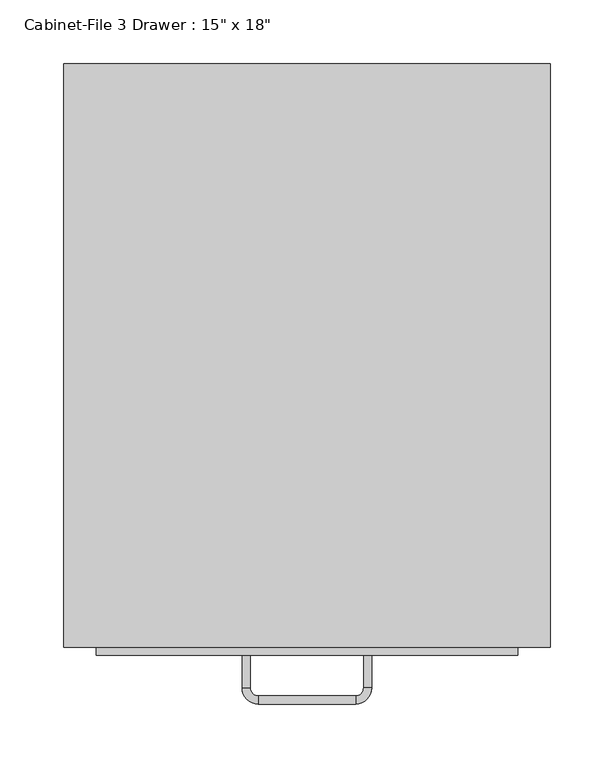
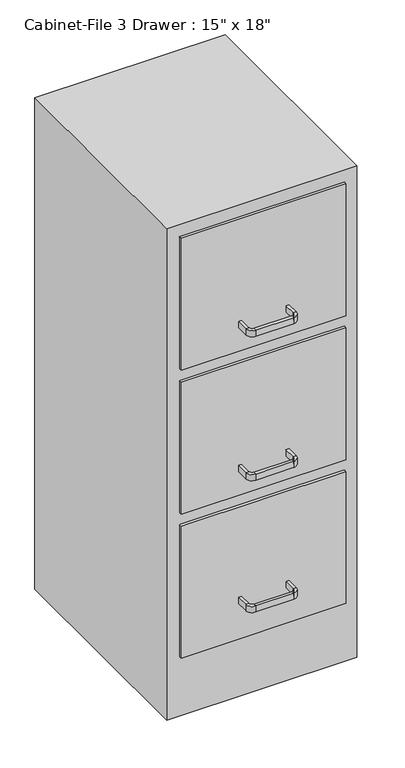
"""IFC4 building model written with IfcOpenShell, lengths in millimetres: furniture geometry."""

import ifcopenshell
import ifcopenshell.guid

model = None  # the IFC model being written
_history = None  # IfcOwnerHistory: only IFC2X3 demands one
_inside = {}  # id of a spatial element -> (the spatial element, [elements in it])
_under = {}  # id of a project, library or spatial element -> (it, [spatial elements below it])
_declared = {}  # id of a project -> (the project, [libraries it declares])
_typed = {}  # id of a type object -> (the type object, [elements of that type])
_made_of = {}  # id of a material, layer set ... -> (it, [elements and type objects made of it])


def new_model(schema):
    """Start an empty IFC model of exactly this schema.

    Asked for "IFC4X3", IfcOpenShell would pick the latest addendum, in which some entities
    have other attributes; the version numbers below select the first issue.
    IFC2X3 requires an IfcOwnerHistory on every rooted entity: one is made here for all.
    """
    global model, _history
    if schema == "IFC4X3":
        model = ifcopenshell.file(schema_version=(4, 3, 0, 0))
    else:
        model = ifcopenshell.file(schema=schema)
    _inside.clear()
    _under.clear()
    _declared.clear()
    _typed.clear()
    _made_of.clear()
    _history = None
    if model.schema == "IFC2X3":
        org = make("IfcOrganization", Name="unknown")
        user = make(
            "IfcPersonAndOrganization",
            ThePerson=make("IfcPerson", FamilyName="unknown"),
            TheOrganization=org,
        )
        app = make(
            "IfcApplication",
            ApplicationDeveloper=org,
            Version="unknown",
            ApplicationFullName="unknown",
            ApplicationIdentifier="unknown",
        )
        _history = make(
            "IfcOwnerHistory",
            OwningUser=user,
            OwningApplication=app,
            ChangeAction="ADDED",
            CreationDate=0,
        )
    return model


def make(cls, **values):
    """One entity of the class cls with the attributes given. An attribute that is None is left unset."""
    return model.create_entity(
        cls, **{name: value for name, value in values.items() if value is not None}
    )


def rooted(cls, **values):
    """An entity with a GlobalId (a new one), such as an element, a storey or a relation."""
    return make(cls, GlobalId=ifcopenshell.guid.new(), OwnerHistory=_history, **values)


def si_unit(unit_type, name, prefix=None):
    """IfcSIUnit, for example si_unit("LENGTHUNIT", "METRE", prefix="MILLI")."""
    return make("IfcSIUnit", UnitType=unit_type, Prefix=prefix, Name=name)


def assignment(units):
    """IfcUnitAssignment: the units of a project."""
    return None if units is None else make("IfcUnitAssignment", Units=units)


def point(xyz):
    """IfcCartesianPoint."""
    return None if xyz is None else make("IfcCartesianPoint", Coordinates=xyz)


def direction(xyz):
    """IfcDirection."""
    return None if xyz is None else make("IfcDirection", DirectionRatios=xyz)


def frame(location, z_axis=None, x_axis=None):
    """IfcAxis2Placement3D, a coordinate frame: its origin and axes. An axis left out is left unset."""
    return make(
        "IfcAxis2Placement3D",
        Location=point(location),
        Axis=direction(z_axis),
        RefDirection=direction(x_axis),
    )


def origin():
    """The frame at (0, 0, 0) with its axes left unset."""
    return frame((0.0, 0.0, 0.0))


def origin_with_axes():
    """The frame at (0, 0, 0) with the z axis (0, 0, 1) and the x axis (1, 0, 0) written out."""
    return frame((0.0, 0.0, 0.0), z_axis=(0.0, 0.0, 1.0), x_axis=(1.0, 0.0, 0.0))


def place(relative_to, where):
    """IfcLocalPlacement: puts the frame where relative to a parent placement (None: the world)."""
    return make(
        "IfcLocalPlacement", PlacementRelTo=relative_to, RelativePlacement=where
    )


def context(
    kind, dimensions, precision=None, world=None, true_north=None, identifier=None
):
    """IfcGeometricRepresentationContext, for example the 3D "Model" context."""
    return make(
        "IfcGeometricRepresentationContext",
        ContextIdentifier=identifier,
        ContextType=kind,
        CoordinateSpaceDimension=dimensions,
        Precision=precision,
        WorldCoordinateSystem=world,
        TrueNorth=true_north,
    )


def project(units=None, contexts=None):
    """IfcProject with its units and contexts."""
    return rooted(
        "IfcProject",
        Name="project",
        RepresentationContexts=contexts,
        UnitsInContext=assignment(units),
    )


def spatial(cls, under=None, at=None, **own):
    """A site, building, storey or space (cls), placed at a placement, below another one or the project."""
    s = rooted(cls, ObjectPlacement=at, **own)
    if under is not None:
        _under.setdefault(under.id(), (under, []))[1].append(s)
    return s


def polyline(points):
    """IfcPolyline through the points."""
    return make("IfcPolyline", Points=[point(p) for p in points])


def circle_curve(where, radius):
    """IfcCircle in the frame where."""
    return make("IfcCircle", Position=where, Radius=radius)


def outline(outer, holes=None, kind="AREA"):
    """IfcArbitraryClosedProfileDef: a profile drawn as a closed curve; with holes, ...WithVoids."""
    if holes is None:
        return make("IfcArbitraryClosedProfileDef", ProfileType=kind, OuterCurve=outer)
    return make(
        "IfcArbitraryProfileDefWithVoids",
        ProfileType=kind,
        OuterCurve=outer,
        InnerCurves=holes,
    )


def extrude(swept, where, along, depth):
    """IfcExtrudedAreaSolid: the profile swept, set in the frame where, extruded along a direction by depth."""
    return make(
        "IfcExtrudedAreaSolid",
        SweptArea=swept,
        Position=where,
        ExtrudedDirection=direction(along),
        Depth=depth,
    )


def shape(context_of_items, identifier, shape_type, items):
    """IfcShapeRepresentation: the items that make up one representation, for example the "Body"."""
    return make(
        "IfcShapeRepresentation",
        ContextOfItems=context_of_items,
        RepresentationIdentifier=identifier,
        RepresentationType=shape_type,
        Items=items,
    )


def source(mapping_origin, context_of_items, identifier, shape_type, items):
    """IfcRepresentationMap: a shape defined once, which mapped items show again and again."""
    return make(
        "IfcRepresentationMap",
        MappingOrigin=mapping_origin,
        MappedRepresentation=shape(context_of_items, identifier, shape_type, items),
    )


def transform(
    local_origin,
    x_axis=None,
    y_axis=None,
    z_axis=None,
    scale=None,
    scale2=None,
    scale3=None,
    uniform=True,
):
    """IfcCartesianTransformationOperator3D, or its non-uniform kind. x_axis, y_axis, z_axis: its Axis1, 2, 3."""
    if uniform:
        return make(
            "IfcCartesianTransformationOperator3D",
            Axis1=direction(x_axis),
            Axis2=direction(y_axis),
            LocalOrigin=point(local_origin),
            Scale=scale,
            Axis3=direction(z_axis),
        )
    return make(
        "IfcCartesianTransformationOperator3DnonUniform",
        Axis1=direction(x_axis),
        Axis2=direction(y_axis),
        LocalOrigin=point(local_origin),
        Scale=scale,
        Axis3=direction(z_axis),
        Scale2=scale2,
        Scale3=scale3,
    )


def mapped(mapping_source, mapping_target):
    """IfcMappedItem: shows the shape of a source again, moved by a transform."""
    return make(
        "IfcMappedItem", MappingSource=mapping_source, MappingTarget=mapping_target
    )


def made_of(thing, what):
    """Note that an element or type object is made of a material, layer set ...; save() writes the relation."""
    if what is not None:
        _made_of.setdefault(what.id(), (what, []))[1].append(thing)
    return thing


def element(
    cls,
    number,
    at=None,
    inside=None,
    cuts=None,
    type_object=None,
    material=None,
    context=None,
    identifier="Body",
    shape_type=None,
    held_by="IfcProductDefinitionShape",
    body=None,
    shapes=None,
    **own,
):
    """One element of the class cls, such as IfcWall. Its Tag is "e" and its number.

    at: its placement. inside: the storey or other place that contains it. cuts: it is an
    opening in that element (IfcRelVoidsElement). A single representation is given by context,
    identifier, shape_type and body (its items); several are given by shapes. held_by: the class
    of the entity that holds the representations. save() writes the other relations.
    """
    e = rooted(cls, Tag="e%d" % number, ObjectPlacement=at, **own)
    if body is not None:
        shapes = [shape(context, identifier, shape_type, body)]
    if shapes is not None:
        e.Representation = make(held_by, Representations=shapes)
    if inside is not None:
        _inside.setdefault(inside.id(), (inside, []))[1].append(e)
    if cuts is not None:
        rooted(
            "IfcRelVoidsElement", RelatingBuildingElement=cuts, RelatedOpeningElement=e
        )
    if type_object is not None:
        _typed.setdefault(type_object.id(), (type_object, []))[1].append(e)
    return made_of(e, material)


def aggregate(whole, parts):
    """IfcRelAggregates: a whole, such as a stair, and the parts it consists of."""
    return rooted("IfcRelAggregates", RelatingObject=whole, RelatedObjects=parts)


def save(model, path):
    """Write the relations noted so far, then the file.

    IfcRelAggregates (storeys below a building ...), IfcRelContainedInSpatialStructure (elements
    in a storey), IfcRelDefinesByType, IfcRelAssociatesMaterial and IfcRelDeclares: one each for
    every whole, place, type object, material and project.
    """
    for whole, parts in _under.values():
        aggregate(whole, parts)
    for where, things in _inside.values():
        rooted(
            "IfcRelContainedInSpatialStructure",
            RelatedElements=things,
            RelatingStructure=where,
        )
    for kind, things in _typed.values():
        rooted("IfcRelDefinesByType", RelatedObjects=things, RelatingType=kind)
    for what, things in _made_of.values():
        rooted("IfcRelAssociatesMaterial", RelatedObjects=things, RelatingMaterial=what)
    for by, libraries in _declared.values():
        rooted("IfcRelDeclares", RelatingContext=by, RelatedDefinitions=libraries)
    model.write(path)


def plane_surface(at):
    """IfcPlane: the flat surface through the origin of the frame at, square to its z axis."""
    return make("IfcPlane", Position=at)


def cylinder_surface(at, radius):
    """IfcCylindricalSurface: all points at the distance radius from the z axis of the frame at."""
    return make("IfcCylindricalSurface", Position=at, Radius=radius)


def revolved_surface(curve, axis_point, axis_direction):
    """IfcSurfaceOfRevolution: the curve turned about the line through axis_point along axis_direction."""
    return make(
        "IfcSurfaceOfRevolution",
        SweptCurve=make("IfcArbitraryOpenProfileDef", ProfileType="CURVE", Curve=curve),
        AxisPosition=make("IfcAxis1Placement", Location=point(axis_point), Axis=direction(axis_direction)),
    )


def advanced_brep(points, edges, surfaces, faces):
    """IfcAdvancedBrep: a solid bounded by faces that lie on surfaces and meet in shared edges.

    An edge is (start, end): straight between two places in points (the first is 0);
    or (start, end, curve); or (start, end, curve, False) where it runs against its curve.
    A face is (place in surfaces, loops), or (place, loops, False) where it looks against
    its surface's normal. A loop lists edges by number (the first is 1), with a minus sign
    where the edge is run from its end to its start. The first loop is the outer one.
    """
    corners = [point(p) for p in points]
    vertices = [make("IfcVertexPoint", VertexGeometry=c) for c in corners]
    made = []
    for start, end, *more in edges:
        made.append(
            make(
                "IfcEdgeCurve",
                EdgeStart=vertices[start],
                EdgeEnd=vertices[end],
                EdgeGeometry=more[0] if more else make("IfcPolyline", Points=[corners[start], corners[end]]),
                SameSense=more[1] if len(more) > 1 else True,
            )
        )
    hull = []
    for where, loops, *sense in faces:
        bounds = []
        for j, loop in enumerate(loops):
            ring = [make("IfcOrientedEdge", EdgeElement=made[abs(k) - 1], Orientation=k > 0) for k in loop]
            bounds.append(
                make(
                    "IfcFaceOuterBound" if j == 0 else "IfcFaceBound",
                    Bound=make("IfcEdgeLoop", EdgeList=ring),
                    Orientation=True,
                )
            )
        hull.append(make("IfcAdvancedFace", Bounds=bounds, FaceSurface=surfaces[where], SameSense=sense[0] if sense else True))
    return make("IfcAdvancedBrep", Outer=make("IfcClosedShell", CfsFaces=hull))


def furniture_552c1472(model_context):
    return source(origin(), model_context, "Body", "SolidModel", [
        extrude(outline(polyline([(62.603553, 86.4656999), (62.603553, -370.7343001), (-318.396447, -370.7343001), (-318.396447, 86.4656999), (62.603553, 86.4656999)])), origin_with_axes(), (0.0, 0.0, 1.0), 1041.4),
        extrude(outline(polyline([(37.203553, -377.0843001), (-292.996447, -377.0843001), (-292.996447, -370.7343001), (37.203553, -370.7343001), (37.203553, -377.0843001)])), frame((0.0, 0.0, 736.6), z_axis=(0.0, 0.0, 1.0), x_axis=(1.0, 0.0, 0.0)), (0.0, 0.0, 1.0), 279.4),
        extrude(outline(polyline([(37.203553, -377.0843001), (-292.996447, -377.0843001), (-292.996447, -370.7343001), (37.203553, -370.7343001), (37.203553, -377.0843001)])), frame((0.0, 0.0, 431.8), z_axis=(0.0, 0.0, 1.0), x_axis=(1.0, 0.0, 0.0)), (0.0, 0.0, 1.0), 279.4),
        extrude(outline(polyline([(37.203553, -377.0843001), (-292.996447, -377.0843001), (-292.996447, -370.7343001), (37.203553, -370.7343001), (37.203553, -377.0843001)])), frame((0.0, 0.0, 127.0), z_axis=(0.0, 0.0, 1.0), x_axis=(1.0, 0.0, 0.0)), (0.0, 0.0, 1.0), 279.4),
        advanced_brep(
        [(-172.346447, -377.0843001, 203.2), (-178.696447, -377.0843001, 203.2), (-178.696447, -377.0843001, 215.9), (-172.346447, -377.0843001, 215.9), (-172.346447, -402.4843001, 203.2), (-178.696447, -402.4843001, 203.2), (-178.696447, -402.4843001, 215.9), (-172.346447, -402.4843001, 215.9), (-165.996447, -415.1843001, 203.2), (-165.996447, -408.8343001, 203.2), (-165.996447, -415.1843001, 215.9), (-165.996447, -408.8343001, 215.9), (-89.796447, -408.8343001, 203.2), (-89.796447, -415.1843001, 203.2), (-89.796447, -415.1843001, 215.9), (-89.796447, -408.8343001, 215.9), (-77.096447, -402.4843001, 203.2), (-83.446447, -402.4843001, 203.2), (-77.096447, -402.4843001, 215.9), (-83.446447, -402.4843001, 215.9), (-83.446447, -377.0843001, 203.2), (-83.446447, -377.0843001, 215.9), (-77.096447, -377.0843001, 215.9), (-77.096447, -377.0843001, 203.2)],
        [
            (0, 1),
            (1, 2),
            (2, 3),
            (3, 0),
            (0, 4),
            (4, 5),
            (5, 1),
            (5, 6),
            (6, 2),
            (6, 7),
            (7, 3),
            (7, 4),
            (8, 5, circle_curve(frame((-165.996447, -402.4843001, 203.2), z_axis=(0.0, 0.0, -1.0), x_axis=(-1.0, 0.0, 0.0)), 12.7)),
            (4, 9, circle_curve(frame((-165.996447, -402.4843001, 203.2), z_axis=(0.0, 0.0, 1.0), x_axis=(-1.0, 0.0, 0.0)), 6.35)),
            (9, 8),
            (10, 6, circle_curve(frame((-165.996447, -402.4843001, 215.9), z_axis=(0.0, 0.0, -1.0), x_axis=(-1.0, 0.0, 0.0)), 12.7)),
            (8, 10),
            (11, 7, circle_curve(frame((-165.996447, -402.4843001, 215.9), z_axis=(0.0, 0.0, -1.0), x_axis=(-1.0, 0.0, 0.0)), 6.35)),
            (10, 11),
            (11, 9),
            (9, 12),
            (12, 13),
            (13, 8),
            (13, 14),
            (14, 10),
            (14, 15),
            (15, 11),
            (15, 12),
            (16, 13, circle_curve(frame((-89.796447, -402.4843001, 203.2), z_axis=(0.0, 0.0, -1.0), x_axis=(0.0, -1.0, 0.0)), 12.7)),
            (12, 17, circle_curve(frame((-89.796447, -402.4843001, 203.2), z_axis=(0.0, 0.0, 1.0), x_axis=(0.0, -1.0, 0.0)), 6.35)),
            (17, 16),
            (18, 14, circle_curve(frame((-89.796447, -402.4843001, 215.9), z_axis=(0.0, 0.0, -1.0), x_axis=(0.0, -1.0, 0.0)), 12.7)),
            (16, 18),
            (19, 15, circle_curve(frame((-89.796447, -402.4843001, 215.9), z_axis=(0.0, 0.0, -1.0), x_axis=(0.0, -1.0, 0.0)), 6.35)),
            (18, 19),
            (19, 17),
            (20, 21),
            (21, 22),
            (22, 23),
            (23, 20),
            (17, 20),
            (23, 16),
            (22, 18),
            (21, 19),
        ],
        [
            plane_surface(frame((-978.8216451, -377.0843001, 0.0), z_axis=(0.0, 1.0, 0.0), x_axis=(0.0, 0.0, -1.0))),
            plane_surface(frame((-172.346447, -377.0843001, 203.2), z_axis=(0.0, 0.0, -1.0), x_axis=(0.0, -1.0, 0.0))),
            plane_surface(frame((-178.696447, -377.0843001, 203.2), z_axis=(-1.0, 0.0, 0.0), x_axis=(0.0, -1.0, 0.0))),
            plane_surface(frame((-178.696447, -377.0843001, 215.9), z_axis=(0.0, 0.0, 1.0), x_axis=(0.0, -1.0, 0.0))),
            plane_surface(frame((-172.346447, -377.0843001, 215.9), z_axis=(1.0, 0.0, 0.0), x_axis=(0.0, -1.0, 0.0))),
            plane_surface(frame((-165.996447, -402.4843001, 203.2), z_axis=(0.0, 0.0, -1.0), x_axis=(-1.0, 0.0, 0.0))),
            cylinder_surface(frame((-165.996447, -402.4843001, 0.0), z_axis=(0.0, 0.0, 1.0), x_axis=(-1.0, 0.0, 0.0)), 12.7),
            plane_surface(frame((-165.996447, -402.4843001, 215.9), z_axis=(0.0, 0.0, 1.0), x_axis=(-1.0, 0.0, 0.0))),
            revolved_surface(polyline([(-172.34644699999998, -402.4843001, 215.9), (-172.34644699999998, -402.4843001, 203.2)]), (-165.996447, -402.4843001, 0.0), (0.0, 0.0, 1.0)),
            plane_surface(frame((-165.996447, -408.8343001, 203.2), z_axis=(0.0, 0.0, -1.0), x_axis=(1.0, 0.0, 0.0))),
            plane_surface(frame((-165.996447, -415.1843001, 203.2), z_axis=(0.0, -1.0, 0.0), x_axis=(1.0, 0.0, 0.0))),
            plane_surface(frame((-165.996447, -415.1843001, 215.9), z_axis=(0.0, 0.0, 1.0), x_axis=(1.0, 0.0, 0.0))),
            plane_surface(frame((-165.996447, -408.8343001, 215.9), z_axis=(0.0, 1.0, 0.0), x_axis=(1.0, 0.0, 0.0))),
            plane_surface(frame((-89.796447, -402.4843001, 203.2), z_axis=(0.0, 0.0, -1.0), x_axis=(0.0, -1.0, 0.0))),
            cylinder_surface(frame((-89.796447, -402.4843001, 0.0), z_axis=(0.0, 0.0, 1.0), x_axis=(0.0, -1.0, 0.0)), 12.7),
            plane_surface(frame((-89.796447, -402.4843001, 215.9), z_axis=(0.0, 0.0, 1.0), x_axis=(0.0, -1.0, 0.0))),
            revolved_surface(polyline([(-89.796447, -408.8343001, 215.9), (-89.796447, -408.8343001, 203.2)]), (-89.796447, -402.4843001, 0.0), (0.0, 0.0, 1.0)),
            plane_surface(frame((-877.2216451, -377.0843001, 0.0), z_axis=(0.0, 1.0, 0.0), x_axis=(0.0, 0.0, 1.0))),
            plane_surface(frame((-83.446447, -402.4843001, 203.2), z_axis=(0.0, 0.0, -1.0), x_axis=(0.0, 1.0, 0.0))),
            plane_surface(frame((-77.096447, -402.4843001, 203.2), z_axis=(1.0, 0.0, 0.0), x_axis=(0.0, 1.0, 0.0))),
            plane_surface(frame((-77.096447, -402.4843001, 215.9), z_axis=(0.0, 0.0, 1.0), x_axis=(0.0, 1.0, 0.0))),
            plane_surface(frame((-83.446447, -402.4843001, 215.9), z_axis=(-1.0, 0.0, 0.0), x_axis=(0.0, 1.0, 0.0))),
        ],
        [
            (0, [[1, 2, 3, 4]]),
            (1, [[-1, 5, 6, 7]]),
            (2, [[-2, -7, 8, 9]]),
            (3, [[-3, -9, 10, 11]]),
            (4, [[-4, -11, 12, -5]]),
            (5, [[13, -6, 14, 15]]),
            (6, [[16, -8, -13, 17]]),
            (7, [[18, -10, -16, 19]]),
            (8, [[-14, -12, -18, 20]]),
            (9, [[-15, 21, 22, 23]]),
            (10, [[-17, -23, 24, 25]]),
            (11, [[-19, -25, 26, 27]]),
            (12, [[-20, -27, 28, -21]]),
            (13, [[29, -22, 30, 31]]),
            (14, [[32, -24, -29, 33]]),
            (15, [[34, -26, -32, 35]]),
            (16, [[-30, -28, -34, 36]]),
            (17, [[37, 38, 39, 40]]),
            (18, [[-31, 41, -40, 42]]),
            (19, [[-33, -42, -39, 43]]),
            (20, [[-35, -43, -38, 44]]),
            (21, [[-36, -44, -37, -41]]),
        ],
    ),
        advanced_brep(
        [(-172.346447, -377.0843001, 482.6), (-178.696447, -377.0843001, 482.6), (-178.696447, -377.0843001, 495.3), (-172.346447, -377.0843001, 495.3), (-172.346447, -402.4843001, 482.6), (-178.696447, -402.4843001, 482.6), (-178.696447, -402.4843001, 495.3), (-172.346447, -402.4843001, 495.3), (-165.996447, -415.1843001, 482.6), (-165.996447, -408.8343001, 482.6), (-165.996447, -415.1843001, 495.3), (-165.996447, -408.8343001, 495.3), (-89.796447, -408.8343001, 482.6), (-89.796447, -415.1843001, 482.6), (-89.796447, -415.1843001, 495.3), (-89.796447, -408.8343001, 495.3), (-77.096447, -402.4843001, 482.6), (-83.446447, -402.4843001, 482.6), (-77.096447, -402.4843001, 495.3), (-83.446447, -402.4843001, 495.3), (-83.446447, -377.0843001, 482.6), (-83.446447, -377.0843001, 495.3), (-77.096447, -377.0843001, 495.3), (-77.096447, -377.0843001, 482.6)],
        [
            (0, 1),
            (1, 2),
            (2, 3),
            (3, 0),
            (0, 4),
            (4, 5),
            (5, 1),
            (5, 6),
            (6, 2),
            (6, 7),
            (7, 3),
            (7, 4),
            (8, 5, circle_curve(frame((-165.996447, -402.4843001, 482.6), z_axis=(0.0, 0.0, -1.0), x_axis=(-1.0, 0.0, 0.0)), 12.7)),
            (4, 9, circle_curve(frame((-165.996447, -402.4843001, 482.6), z_axis=(0.0, 0.0, 1.0), x_axis=(-1.0, 0.0, 0.0)), 6.35)),
            (9, 8),
            (10, 6, circle_curve(frame((-165.996447, -402.4843001, 495.3), z_axis=(0.0, 0.0, -1.0), x_axis=(-1.0, 0.0, 0.0)), 12.7)),
            (8, 10),
            (11, 7, circle_curve(frame((-165.996447, -402.4843001, 495.3), z_axis=(0.0, 0.0, -1.0), x_axis=(-1.0, 0.0, 0.0)), 6.35)),
            (10, 11),
            (11, 9),
            (9, 12),
            (12, 13),
            (13, 8),
            (13, 14),
            (14, 10),
            (14, 15),
            (15, 11),
            (15, 12),
            (16, 13, circle_curve(frame((-89.796447, -402.4843001, 482.6), z_axis=(0.0, 0.0, -1.0), x_axis=(0.0, -1.0, 0.0)), 12.7)),
            (12, 17, circle_curve(frame((-89.796447, -402.4843001, 482.6), z_axis=(0.0, 0.0, 1.0), x_axis=(0.0, -1.0, 0.0)), 6.35)),
            (17, 16),
            (18, 14, circle_curve(frame((-89.796447, -402.4843001, 495.3), z_axis=(0.0, 0.0, -1.0), x_axis=(0.0, -1.0, 0.0)), 12.7)),
            (16, 18),
            (19, 15, circle_curve(frame((-89.796447, -402.4843001, 495.3), z_axis=(0.0, 0.0, -1.0), x_axis=(0.0, -1.0, 0.0)), 6.35)),
            (18, 19),
            (19, 17),
            (20, 21),
            (21, 22),
            (22, 23),
            (23, 20),
            (17, 20),
            (23, 16),
            (22, 18),
            (21, 19),
        ],
        [
            plane_surface(frame((-978.8216451, -377.0843001, 0.0), z_axis=(0.0, 1.0, 0.0), x_axis=(0.0, 0.0, -1.0))),
            plane_surface(frame((-172.346447, -377.0843001, 482.6), z_axis=(0.0, 0.0, -1.0), x_axis=(0.0, -1.0, 0.0))),
            plane_surface(frame((-178.696447, -377.0843001, 482.6), z_axis=(-1.0, 0.0, 0.0), x_axis=(0.0, -1.0, 0.0))),
            plane_surface(frame((-178.696447, -377.0843001, 495.3), z_axis=(0.0, 0.0, 1.0), x_axis=(0.0, -1.0, 0.0))),
            plane_surface(frame((-172.346447, -377.0843001, 495.3), z_axis=(1.0, 0.0, 0.0), x_axis=(0.0, -1.0, 0.0))),
            plane_surface(frame((-165.996447, -402.4843001, 482.6), z_axis=(0.0, 0.0, -1.0), x_axis=(-1.0, 0.0, 0.0))),
            cylinder_surface(frame((-165.996447, -402.4843001, 0.0), z_axis=(0.0, 0.0, 1.0), x_axis=(-1.0, 0.0, 0.0)), 12.7),
            plane_surface(frame((-165.996447, -402.4843001, 495.3), z_axis=(0.0, 0.0, 1.0), x_axis=(-1.0, 0.0, 0.0))),
            revolved_surface(polyline([(-172.34644699999998, -402.4843001, 495.3), (-172.34644699999998, -402.4843001, 482.6)]), (-165.996447, -402.4843001, 0.0), (0.0, 0.0, 1.0)),
            plane_surface(frame((-165.996447, -408.8343001, 482.6), z_axis=(0.0, 0.0, -1.0), x_axis=(1.0, 0.0, 0.0))),
            plane_surface(frame((-165.996447, -415.1843001, 482.6), z_axis=(0.0, -1.0, 0.0), x_axis=(1.0, 0.0, 0.0))),
            plane_surface(frame((-165.996447, -415.1843001, 495.3), z_axis=(0.0, 0.0, 1.0), x_axis=(1.0, 0.0, 0.0))),
            plane_surface(frame((-165.996447, -408.8343001, 495.3), z_axis=(0.0, 1.0, 0.0), x_axis=(1.0, 0.0, 0.0))),
            plane_surface(frame((-89.796447, -402.4843001, 482.6), z_axis=(0.0, 0.0, -1.0), x_axis=(0.0, -1.0, 0.0))),
            cylinder_surface(frame((-89.796447, -402.4843001, 0.0), z_axis=(0.0, 0.0, 1.0), x_axis=(0.0, -1.0, 0.0)), 12.7),
            plane_surface(frame((-89.796447, -402.4843001, 495.3), z_axis=(0.0, 0.0, 1.0), x_axis=(0.0, -1.0, 0.0))),
            revolved_surface(polyline([(-89.796447, -408.8343001, 495.3), (-89.796447, -408.8343001, 482.6)]), (-89.796447, -402.4843001, 0.0), (0.0, 0.0, 1.0)),
            plane_surface(frame((-877.2216451, -377.0843001, 0.0), z_axis=(0.0, 1.0, 0.0), x_axis=(0.0, 0.0, 1.0))),
            plane_surface(frame((-83.446447, -402.4843001, 482.6), z_axis=(0.0, 0.0, -1.0), x_axis=(0.0, 1.0, 0.0))),
            plane_surface(frame((-77.096447, -402.4843001, 482.6), z_axis=(1.0, 0.0, 0.0), x_axis=(0.0, 1.0, 0.0))),
            plane_surface(frame((-77.096447, -402.4843001, 495.3), z_axis=(0.0, 0.0, 1.0), x_axis=(0.0, 1.0, 0.0))),
            plane_surface(frame((-83.446447, -402.4843001, 495.3), z_axis=(-1.0, 0.0, 0.0), x_axis=(0.0, 1.0, 0.0))),
        ],
        [
            (0, [[1, 2, 3, 4]]),
            (1, [[-1, 5, 6, 7]]),
            (2, [[-2, -7, 8, 9]]),
            (3, [[-3, -9, 10, 11]]),
            (4, [[-4, -11, 12, -5]]),
            (5, [[13, -6, 14, 15]]),
            (6, [[16, -8, -13, 17]]),
            (7, [[18, -10, -16, 19]]),
            (8, [[-14, -12, -18, 20]]),
            (9, [[-15, 21, 22, 23]]),
            (10, [[-17, -23, 24, 25]]),
            (11, [[-19, -25, 26, 27]]),
            (12, [[-20, -27, 28, -21]]),
            (13, [[29, -22, 30, 31]]),
            (14, [[32, -24, -29, 33]]),
            (15, [[34, -26, -32, 35]]),
            (16, [[-30, -28, -34, 36]]),
            (17, [[37, 38, 39, 40]]),
            (18, [[-31, 41, -40, 42]]),
            (19, [[-33, -42, -39, 43]]),
            (20, [[-35, -43, -38, 44]]),
            (21, [[-36, -44, -37, -41]]),
        ],
    ),
        advanced_brep(
        [(-172.346447, -377.0843001, 787.4), (-178.696447, -377.0843001, 787.4), (-178.696447, -377.0843001, 800.1), (-172.346447, -377.0843001, 800.1), (-172.346447, -402.4843001, 787.4), (-178.696447, -402.4843001, 787.4), (-178.696447, -402.4843001, 800.1), (-172.346447, -402.4843001, 800.1), (-165.996447, -415.1843001, 787.4), (-165.996447, -408.8343001, 787.4), (-165.996447, -415.1843001, 800.1), (-165.996447, -408.8343001, 800.1), (-89.796447, -408.8343001, 787.4), (-89.796447, -415.1843001, 787.4), (-89.796447, -415.1843001, 800.1), (-89.796447, -408.8343001, 800.1), (-77.096447, -402.4843001, 787.4), (-83.446447, -402.4843001, 787.4), (-77.096447, -402.4843001, 800.1), (-83.446447, -402.4843001, 800.1), (-83.446447, -377.0843001, 787.4), (-83.446447, -377.0843001, 800.1), (-77.096447, -377.0843001, 800.1), (-77.096447, -377.0843001, 787.4)],
        [
            (0, 1),
            (1, 2),
            (2, 3),
            (3, 0),
            (0, 4),
            (4, 5),
            (5, 1),
            (5, 6),
            (6, 2),
            (6, 7),
            (7, 3),
            (7, 4),
            (8, 5, circle_curve(frame((-165.996447, -402.4843001, 787.4), z_axis=(0.0, 0.0, -1.0), x_axis=(-1.0, 0.0, 0.0)), 12.7)),
            (4, 9, circle_curve(frame((-165.996447, -402.4843001, 787.4), z_axis=(0.0, 0.0, 1.0), x_axis=(-1.0, 0.0, 0.0)), 6.35)),
            (9, 8),
            (10, 6, circle_curve(frame((-165.996447, -402.4843001, 800.1), z_axis=(0.0, 0.0, -1.0), x_axis=(-1.0, 0.0, 0.0)), 12.7)),
            (8, 10),
            (11, 7, circle_curve(frame((-165.996447, -402.4843001, 800.1), z_axis=(0.0, 0.0, -1.0), x_axis=(-1.0, 0.0, 0.0)), 6.35)),
            (10, 11),
            (11, 9),
            (9, 12),
            (12, 13),
            (13, 8),
            (13, 14),
            (14, 10),
            (14, 15),
            (15, 11),
            (15, 12),
            (16, 13, circle_curve(frame((-89.796447, -402.4843001, 787.4), z_axis=(0.0, 0.0, -1.0), x_axis=(0.0, -1.0, 0.0)), 12.7)),
            (12, 17, circle_curve(frame((-89.796447, -402.4843001, 787.4), z_axis=(0.0, 0.0, 1.0), x_axis=(0.0, -1.0, 0.0)), 6.35)),
            (17, 16),
            (18, 14, circle_curve(frame((-89.796447, -402.4843001, 800.1), z_axis=(0.0, 0.0, -1.0), x_axis=(0.0, -1.0, 0.0)), 12.7)),
            (16, 18),
            (19, 15, circle_curve(frame((-89.796447, -402.4843001, 800.1), z_axis=(0.0, 0.0, -1.0), x_axis=(0.0, -1.0, 0.0)), 6.35)),
            (18, 19),
            (19, 17),
            (20, 21),
            (21, 22),
            (22, 23),
            (23, 20),
            (17, 20),
            (23, 16),
            (22, 18),
            (21, 19),
        ],
        [
            plane_surface(frame((-978.8216451, -377.0843001, 0.0), z_axis=(0.0, 1.0, 0.0), x_axis=(0.0, 0.0, -1.0))),
            plane_surface(frame((-172.346447, -377.0843001, 787.4), z_axis=(0.0, 0.0, -1.0), x_axis=(0.0, -1.0, 0.0))),
            plane_surface(frame((-178.696447, -377.0843001, 787.4), z_axis=(-1.0, 0.0, 0.0), x_axis=(0.0, -1.0, 0.0))),
            plane_surface(frame((-178.696447, -377.0843001, 800.1), z_axis=(0.0, 0.0, 1.0), x_axis=(0.0, -1.0, 0.0))),
            plane_surface(frame((-172.346447, -377.0843001, 800.1), z_axis=(1.0, 0.0, 0.0), x_axis=(0.0, -1.0, 0.0))),
            plane_surface(frame((-165.996447, -402.4843001, 787.4), z_axis=(0.0, 0.0, -1.0), x_axis=(-1.0, 0.0, 0.0))),
            cylinder_surface(frame((-165.996447, -402.4843001, 0.0), z_axis=(0.0, 0.0, 1.0), x_axis=(-1.0, 0.0, 0.0)), 12.7),
            plane_surface(frame((-165.996447, -402.4843001, 800.1), z_axis=(0.0, 0.0, 1.0), x_axis=(-1.0, 0.0, 0.0))),
            revolved_surface(polyline([(-172.34644699999998, -402.4843001, 800.1), (-172.34644699999998, -402.4843001, 787.4)]), (-165.996447, -402.4843001, 0.0), (0.0, 0.0, 1.0)),
            plane_surface(frame((-165.996447, -408.8343001, 787.4), z_axis=(0.0, 0.0, -1.0), x_axis=(1.0, 0.0, 0.0))),
            plane_surface(frame((-165.996447, -415.1843001, 787.4), z_axis=(0.0, -1.0, 0.0), x_axis=(1.0, 0.0, 0.0))),
            plane_surface(frame((-165.996447, -415.1843001, 800.1), z_axis=(0.0, 0.0, 1.0), x_axis=(1.0, 0.0, 0.0))),
            plane_surface(frame((-165.996447, -408.8343001, 800.1), z_axis=(0.0, 1.0, 0.0), x_axis=(1.0, 0.0, 0.0))),
            plane_surface(frame((-89.796447, -402.4843001, 787.4), z_axis=(0.0, 0.0, -1.0), x_axis=(0.0, -1.0, 0.0))),
            cylinder_surface(frame((-89.796447, -402.4843001, 0.0), z_axis=(0.0, 0.0, 1.0), x_axis=(0.0, -1.0, 0.0)), 12.7),
            plane_surface(frame((-89.796447, -402.4843001, 800.1), z_axis=(0.0, 0.0, 1.0), x_axis=(0.0, -1.0, 0.0))),
            revolved_surface(polyline([(-89.796447, -408.8343001, 800.1), (-89.796447, -408.8343001, 787.4)]), (-89.796447, -402.4843001, 0.0), (0.0, 0.0, 1.0)),
            plane_surface(frame((-877.2216451, -377.0843001, 0.0), z_axis=(0.0, 1.0, 0.0), x_axis=(0.0, 0.0, 1.0))),
            plane_surface(frame((-83.446447, -402.4843001, 787.4), z_axis=(0.0, 0.0, -1.0), x_axis=(0.0, 1.0, 0.0))),
            plane_surface(frame((-77.096447, -402.4843001, 787.4), z_axis=(1.0, 0.0, 0.0), x_axis=(0.0, 1.0, 0.0))),
            plane_surface(frame((-77.096447, -402.4843001, 800.1), z_axis=(0.0, 0.0, 1.0), x_axis=(0.0, 1.0, 0.0))),
            plane_surface(frame((-83.446447, -402.4843001, 800.1), z_axis=(-1.0, 0.0, 0.0), x_axis=(0.0, 1.0, 0.0))),
        ],
        [
            (0, [[1, 2, 3, 4]]),
            (1, [[-1, 5, 6, 7]]),
            (2, [[-2, -7, 8, 9]]),
            (3, [[-3, -9, 10, 11]]),
            (4, [[-4, -11, 12, -5]]),
            (5, [[13, -6, 14, 15]]),
            (6, [[16, -8, -13, 17]]),
            (7, [[18, -10, -16, 19]]),
            (8, [[-14, -12, -18, 20]]),
            (9, [[-15, 21, 22, 23]]),
            (10, [[-17, -23, 24, 25]]),
            (11, [[-19, -25, 26, 27]]),
            (12, [[-20, -27, 28, -21]]),
            (13, [[29, -22, 30, 31]]),
            (14, [[32, -24, -29, 33]]),
            (15, [[34, -26, -32, 35]]),
            (16, [[-30, -28, -34, 36]]),
            (17, [[37, 38, 39, 40]]),
            (18, [[-31, 41, -40, 42]]),
            (19, [[-33, -42, -39, 43]]),
            (20, [[-35, -43, -38, 44]]),
            (21, [[-36, -44, -37, -41]]),
        ],
    ),
    ])


if __name__ == "__main__":
    model = new_model("IFC4")
    model_context = context("Model", 3, world=origin())
    ifc_project = project(units=[si_unit("LENGTHUNIT", "METRE", prefix="MILLI")], contexts=[model_context])
    site = spatial("IfcSite", under=ifc_project)
    building = spatial("IfcBuilding", under=site)
    placement = place(None, origin())
    furniture_shape = furniture_552c1472(model_context)
    element("IfcFurniture", 1, ObjectType="Cabinet-File 3 Drawer : 15\" x 18\"", at=placement, inside=building, context=model_context, shape_type="MappedRepresentation", body=[
        mapped(furniture_shape, transform((0.0, 0.0, 0.0), x_axis=(1.0, 0.0, 0.0), y_axis=(0.0, 1.0, 0.0), z_axis=(0.0, 0.0, 1.0))),
    ])
    save(model, "model.ifc")

# Revit data of these elements
# Type "Cabinet-File 3 Drawer : 15\" x 18\""
#   Assembly Code = "E2020200"
#   Depth = 1' - 6"
#   Height = 3' - 5"
#   Width = 1' - 3"
#   Cabinet Material = Steel, Paint Finish, Ivory, Glossy
#   Handle Material = Steel, Chrome Plated
#   Default Elevation = 0
# Element 1 (IfcFurniture, "Cabinet-File 3 Drawer : 15\" x 18\"")
#   Materials on its faces: "Steel, Chrome Plated", "Steel, Paint Finish, Ivory, Glossy"
# Materials
#   "Steel, Paint Finish, Ivory, Glossy": class "Metal", colour RGB 247 247 239, transparency 0, Description = "Steel, paint finish, ivory, glossy", Cost = 0
#   "Steel, Chrome Plated": class "Metal", colour RGB 17 17 17, transparency 0, Description = "Chromiuim plated steel", Cost = 0
